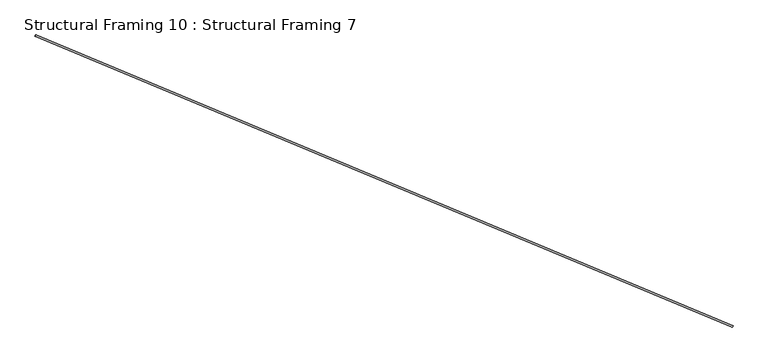
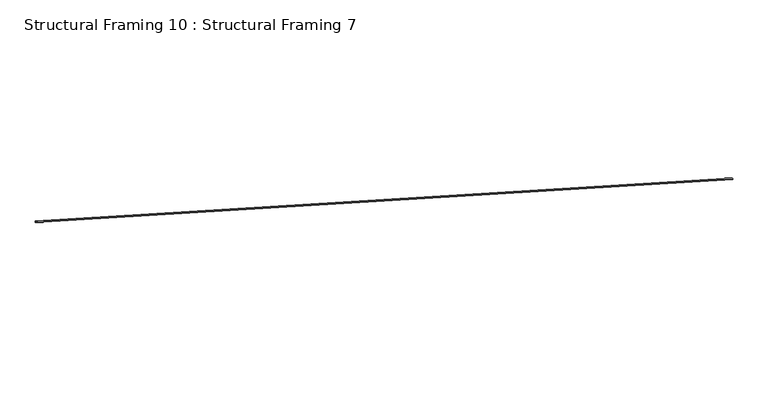
"""IFC4 building model written with IfcOpenShell, lengths in millimetres: beam geometry, Structural Framing 10 : Structural Framing 7."""

import ifcopenshell
import ifcopenshell.guid

model = None  # the IFC model being written
_history = None  # IfcOwnerHistory: only IFC2X3 demands one
_inside = {}  # id of a spatial element -> (the spatial element, [elements in it])
_under = {}  # id of a project, library or spatial element -> (it, [spatial elements below it])
_declared = {}  # id of a project -> (the project, [libraries it declares])
_typed = {}  # id of a type object -> (the type object, [elements of that type])
_made_of = {}  # id of a material, layer set ... -> (it, [elements and type objects made of it])


def new_model(schema):
    """Start an empty IFC model of exactly this schema.

    Asked for "IFC4X3", IfcOpenShell would pick the latest addendum, in which some entities
    have other attributes; the version numbers below select the first issue.
    IFC2X3 requires an IfcOwnerHistory on every rooted entity: one is made here for all.
    """
    global model, _history
    if schema == "IFC4X3":
        model = ifcopenshell.file(schema_version=(4, 3, 0, 0))
    else:
        model = ifcopenshell.file(schema=schema)
    _inside.clear()
    _under.clear()
    _declared.clear()
    _typed.clear()
    _made_of.clear()
    _history = None
    if model.schema == "IFC2X3":
        org = make("IfcOrganization", Name="unknown")
        user = make(
            "IfcPersonAndOrganization",
            ThePerson=make("IfcPerson", FamilyName="unknown"),
            TheOrganization=org,
        )
        app = make(
            "IfcApplication",
            ApplicationDeveloper=org,
            Version="unknown",
            ApplicationFullName="unknown",
            ApplicationIdentifier="unknown",
        )
        _history = make(
            "IfcOwnerHistory",
            OwningUser=user,
            OwningApplication=app,
            ChangeAction="ADDED",
            CreationDate=0,
        )
    return model


def make(cls, **values):
    """One entity of the class cls with the attributes given. An attribute that is None is left unset."""
    return model.create_entity(
        cls, **{name: value for name, value in values.items() if value is not None}
    )


def rooted(cls, **values):
    """An entity with a GlobalId (a new one), such as an element, a storey or a relation."""
    return make(cls, GlobalId=ifcopenshell.guid.new(), OwnerHistory=_history, **values)


def si_unit(unit_type, name, prefix=None):
    """IfcSIUnit, for example si_unit("LENGTHUNIT", "METRE", prefix="MILLI")."""
    return make("IfcSIUnit", UnitType=unit_type, Prefix=prefix, Name=name)


def assignment(units):
    """IfcUnitAssignment: the units of a project."""
    return None if units is None else make("IfcUnitAssignment", Units=units)


def point(xyz):
    """IfcCartesianPoint."""
    return None if xyz is None else make("IfcCartesianPoint", Coordinates=xyz)


def direction(xyz):
    """IfcDirection."""
    return None if xyz is None else make("IfcDirection", DirectionRatios=xyz)


def frame(location, z_axis=None, x_axis=None):
    """IfcAxis2Placement3D, a coordinate frame: its origin and axes. An axis left out is left unset."""
    return make(
        "IfcAxis2Placement3D",
        Location=point(location),
        Axis=direction(z_axis),
        RefDirection=direction(x_axis),
    )


def frame_2d(location, x_axis=None):
    """IfcAxis2Placement2D, a coordinate frame in the plane: its origin and x axis."""
    return make(
        "IfcAxis2Placement2D", Location=point(location), RefDirection=direction(x_axis)
    )


def origin():
    """The frame at (0, 0, 0) with its axes left unset."""
    return frame((0.0, 0.0, 0.0))


def origin_2d():
    """The frame at (0, 0) in the plane with its x axis left unset."""
    return frame_2d((0.0, 0.0))


def place(relative_to, where):
    """IfcLocalPlacement: puts the frame where relative to a parent placement (None: the world)."""
    return make(
        "IfcLocalPlacement", PlacementRelTo=relative_to, RelativePlacement=where
    )


def context(
    kind, dimensions, precision=None, world=None, true_north=None, identifier=None
):
    """IfcGeometricRepresentationContext, for example the 3D "Model" context."""
    return make(
        "IfcGeometricRepresentationContext",
        ContextIdentifier=identifier,
        ContextType=kind,
        CoordinateSpaceDimension=dimensions,
        Precision=precision,
        WorldCoordinateSystem=world,
        TrueNorth=true_north,
    )


def project(units=None, contexts=None):
    """IfcProject with its units and contexts."""
    return rooted(
        "IfcProject",
        Name="project",
        RepresentationContexts=contexts,
        UnitsInContext=assignment(units),
    )


def spatial(cls, under=None, at=None, **own):
    """A site, building, storey or space (cls), placed at a placement, below another one or the project."""
    s = rooted(cls, ObjectPlacement=at, **own)
    if under is not None:
        _under.setdefault(under.id(), (under, []))[1].append(s)
    return s


def circle_curve(where, radius):
    """IfcCircle in the frame where."""
    return make("IfcCircle", Position=where, Radius=radius)


def trimmed(basis, trim1, trim2, sense, master):
    """IfcTrimmedCurve: the piece of a basis curve between two trims."""
    return make(
        "IfcTrimmedCurve",
        BasisCurve=basis,
        Trim1=trim1,
        Trim2=trim2,
        SenseAgreement=sense,
        MasterRepresentation=master,
    )


def segment(curve, same_sense, transition):
    """IfcCompositeCurveSegment."""
    return make(
        "IfcCompositeCurveSegment",
        Transition=transition,
        SameSense=same_sense,
        ParentCurve=curve,
    )


def composite_curve(segments, self_intersect=None):
    """IfcCompositeCurve: segments joined end to end."""
    return make("IfcCompositeCurve", Segments=segments, SelfIntersect=self_intersect)


def outline(outer, holes=None, kind="AREA"):
    """IfcArbitraryClosedProfileDef: a profile drawn as a closed curve; with holes, ...WithVoids."""
    if holes is None:
        return make("IfcArbitraryClosedProfileDef", ProfileType=kind, OuterCurve=outer)
    return make(
        "IfcArbitraryProfileDefWithVoids",
        ProfileType=kind,
        OuterCurve=outer,
        InnerCurves=holes,
    )


def extrude(swept, where, along, depth):
    """IfcExtrudedAreaSolid: the profile swept, set in the frame where, extruded along a direction by depth."""
    return make(
        "IfcExtrudedAreaSolid",
        SweptArea=swept,
        Position=where,
        ExtrudedDirection=direction(along),
        Depth=depth,
    )


def shape(context_of_items, identifier, shape_type, items):
    """IfcShapeRepresentation: the items that make up one representation, for example the "Body"."""
    return make(
        "IfcShapeRepresentation",
        ContextOfItems=context_of_items,
        RepresentationIdentifier=identifier,
        RepresentationType=shape_type,
        Items=items,
    )


def source(mapping_origin, context_of_items, identifier, shape_type, items):
    """IfcRepresentationMap: a shape defined once, which mapped items show again and again."""
    return make(
        "IfcRepresentationMap",
        MappingOrigin=mapping_origin,
        MappedRepresentation=shape(context_of_items, identifier, shape_type, items),
    )


def transform(
    local_origin,
    x_axis=None,
    y_axis=None,
    z_axis=None,
    scale=None,
    scale2=None,
    scale3=None,
    uniform=True,
):
    """IfcCartesianTransformationOperator3D, or its non-uniform kind. x_axis, y_axis, z_axis: its Axis1, 2, 3."""
    if uniform:
        return make(
            "IfcCartesianTransformationOperator3D",
            Axis1=direction(x_axis),
            Axis2=direction(y_axis),
            LocalOrigin=point(local_origin),
            Scale=scale,
            Axis3=direction(z_axis),
        )
    return make(
        "IfcCartesianTransformationOperator3DnonUniform",
        Axis1=direction(x_axis),
        Axis2=direction(y_axis),
        LocalOrigin=point(local_origin),
        Scale=scale,
        Axis3=direction(z_axis),
        Scale2=scale2,
        Scale3=scale3,
    )


def mapped(mapping_source, mapping_target):
    """IfcMappedItem: shows the shape of a source again, moved by a transform."""
    return make(
        "IfcMappedItem", MappingSource=mapping_source, MappingTarget=mapping_target
    )


def made_of(thing, what):
    """Note that an element or type object is made of a material, layer set ...; save() writes the relation."""
    if what is not None:
        _made_of.setdefault(what.id(), (what, []))[1].append(thing)
    return thing


def element(
    cls,
    number,
    at=None,
    inside=None,
    cuts=None,
    type_object=None,
    material=None,
    context=None,
    identifier="Body",
    shape_type=None,
    held_by="IfcProductDefinitionShape",
    body=None,
    shapes=None,
    **own,
):
    """One element of the class cls, such as IfcWall. Its Tag is "e" and its number.

    at: its placement. inside: the storey or other place that contains it. cuts: it is an
    opening in that element (IfcRelVoidsElement). A single representation is given by context,
    identifier, shape_type and body (its items); several are given by shapes. held_by: the class
    of the entity that holds the representations. save() writes the other relations.
    """
    e = rooted(cls, Tag="e%d" % number, ObjectPlacement=at, **own)
    if body is not None:
        shapes = [shape(context, identifier, shape_type, body)]
    if shapes is not None:
        e.Representation = make(held_by, Representations=shapes)
    if inside is not None:
        _inside.setdefault(inside.id(), (inside, []))[1].append(e)
    if cuts is not None:
        rooted(
            "IfcRelVoidsElement", RelatingBuildingElement=cuts, RelatedOpeningElement=e
        )
    if type_object is not None:
        _typed.setdefault(type_object.id(), (type_object, []))[1].append(e)
    return made_of(e, material)


def aggregate(whole, parts):
    """IfcRelAggregates: a whole, such as a stair, and the parts it consists of."""
    return rooted("IfcRelAggregates", RelatingObject=whole, RelatedObjects=parts)


def save(model, path):
    """Write the relations noted so far, then the file.

    IfcRelAggregates (storeys below a building ...), IfcRelContainedInSpatialStructure (elements
    in a storey), IfcRelDefinesByType, IfcRelAssociatesMaterial and IfcRelDeclares: one each for
    every whole, place, type object, material and project.
    """
    for whole, parts in _under.values():
        aggregate(whole, parts)
    for where, things in _inside.values():
        rooted(
            "IfcRelContainedInSpatialStructure",
            RelatedElements=things,
            RelatingStructure=where,
        )
    for kind, things in _typed.values():
        rooted("IfcRelDefinesByType", RelatedObjects=things, RelatingType=kind)
    for what, things in _made_of.values():
        rooted("IfcRelAssociatesMaterial", RelatedObjects=things, RelatingMaterial=what)
    for by, libraries in _declared.values():
        rooted("IfcRelDeclares", RelatingContext=by, RelatedDefinitions=libraries)
    model.write(path)


def structural_framing_10_structural_framing_7_f952438b(model_context):
    return source(origin(), model_context, "Body", "SweptSolid", [
        extrude(outline(composite_curve([segment(trimmed(circle_curve(origin_2d(), 6.35), [point((0.0, 6.35))], [point((0.0, -6.3500001))], False, "CARTESIAN"), True, "CONTINUOUS"), segment(trimmed(circle_curve(origin_2d(), 6.35), [point((0.0, -6.3500001))], [point((0.0, 6.35))], False, "CARTESIAN"), True, "CONTINUOUS")], self_intersect=False)), frame((17937.0897681, 282.3662123, 2861.0177297), z_axis=(-0.9227531257280362, 0.38510091650472056, 0.014965061522204016), x_axis=(0.0, 0.03883079534680305, -0.9992458002577418)), (0.0, 0.0, 1.0), 5780.5276962),
    ])


if __name__ == "__main__":
    model = new_model("IFC4")
    model_context = context("Model", 3, world=origin())
    ifc_project = project(units=[si_unit("LENGTHUNIT", "METRE", prefix="MILLI")], contexts=[model_context])
    site = spatial("IfcSite", under=ifc_project)
    building = spatial("IfcBuilding", under=site)
    placement = place(None, origin())
    structural_framing_10_structural_framing_7_shape = structural_framing_10_structural_framing_7_f952438b(model_context)
    element("IfcBeam", 1, ObjectType="Structural Framing 10 : Structural Framing 7", at=placement, inside=building, context=model_context, shape_type="MappedRepresentation", body=[
        mapped(structural_framing_10_structural_framing_7_shape, transform((0.0, 0.0, 0.0), x_axis=(1.0, 0.0, 0.0), y_axis=(0.0, 1.0, 0.0), z_axis=(0.0, 0.0, 1.0))),
    ])
    save(model, "model.ifc")

# Revit data of these elements
# Type "Structural Framing 10 : Structural Framing 7"
#   Structural Material [instance default] = EXISTING LATERAL BRACING (1/4" CABLE)
# Element 1 (IfcBeam, "Structural Framing 10 : Structural Framing 7")
#   Materials on its faces: "EXISTING LATERAL BRACING (1/4\" CABLE)"
# Materials
#   "EXISTING LATERAL BRACING (1/4\" CABLE)": class "Generic", colour RGB 120 120 120, transparency 0, Cost = 0
